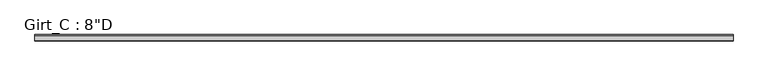
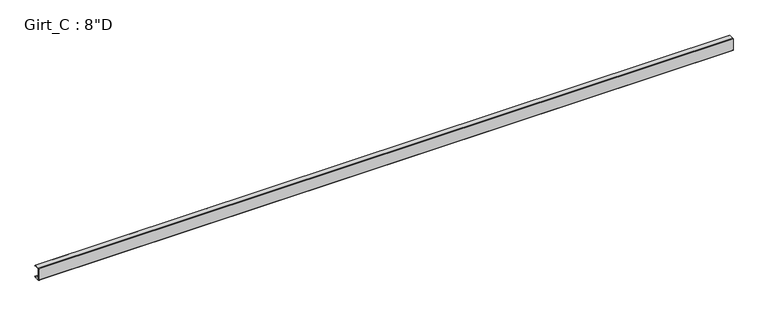
"""IFC4 building model written with IfcOpenShell, lengths in millimetres: beam geometry."""

from ifc_helpers import new_model, si_unit, point, frame, frame_2d, origin, place, context, project, spatial, polyline, circle_curve, trimmed, segment, composite_curve, outline, extrude, source, transform, mapped, element, save


def beam_5935eb23(model_context):
    return source(origin(), model_context, "Body", "SweptSolid", [
        extrude(outline(composite_curve([segment(polyline([(87.5109375, 101.6), (99.7560415, 87.0068534), (97.6278742, 85.221109), (86.2154765, 98.821875), (3.3005807, 98.821875)]), True, "CONTINUOUS"), segment(trimmed(circle_curve(frame_2d((3.3741066, 96.8381931)), 1.9850441), [point((3.3005807, 98.821875))], [point((1.3890625, 96.8381931))], True, "CARTESIAN"), True, "CONTINUOUS"), segment(polyline([(1.3890625, 96.8381931), (1.3890625, -96.8389339)]), True, "CONTINUOUS"), segment(trimmed(circle_curve(frame_2d((3.3748024, -96.8389339)), 1.9857399), [point((1.3890625, -96.8389339))], [point((3.2694106, -98.821875))], True, "CARTESIAN"), True, "CONTINUOUS"), segment(polyline([(3.2694106, -98.821875), (86.2154765, -98.821875), (97.6510975, -85.1934327), (99.7792647, -86.979177), (87.5109375, -101.6), (3.3734375, -101.6)]), True, "CONTINUOUS"), segment(trimmed(circle_curve(frame_2d((3.3734375, -96.8375)), 4.7625), [point((3.3734375, -101.6))], [point((-1.3890625, -96.8375))], False, "CARTESIAN"), True, "CONTINUOUS"), segment(polyline([(-1.3890625, -96.8375), (-1.3890625, 96.8375)]), True, "CONTINUOUS"), segment(trimmed(circle_curve(frame_2d((3.3734375, 96.8375)), 4.7625), [point((-1.3890625, 96.8375))], [point((3.3734375, 101.6))], False, "CARTESIAN"), True, "CONTINUOUS"), segment(polyline([(3.3734375, 101.6), (87.5109375, 101.6)]), True, "CONTINUOUS")], self_intersect=False)), frame((-5621.3960997, 0.0, 0.0), z_axis=(1.0, 0.0, 0.0), x_axis=(0.0, 1.0, 0.0)), (0.0, 0.0, 1.0), 11076.8984495),
    ])


if __name__ == "__main__":
    model = new_model("IFC4")
    model_context = context("Model", 3, world=origin())
    ifc_project = project(units=[si_unit("LENGTHUNIT", "METRE", prefix="MILLI")], contexts=[model_context])
    site = spatial("IfcSite", under=ifc_project)
    building = spatial("IfcBuilding", under=site)
    placement = place(None, origin())
    beam_shape = beam_5935eb23(model_context)
    element("IfcBeam", 1, ObjectType="Girt_C : 8\"D", at=placement, inside=building, context=model_context, shape_type="MappedRepresentation", body=[
        mapped(beam_shape, transform((0.0, 0.0, 0.0), x_axis=(1.0, 0.0, 0.0), y_axis=(0.0, 1.0, 0.0), z_axis=(0.0, 0.0, 1.0))),
    ])
    save(model, "model.ifc")

# Revit data of these elements
# Type "Girt_C : 8\"D"
#   half leg = 0' - 1 3/4"
#   Web_Thickness = 0' - 0 7/64"
#   Length [instance default] = 10' - 0"
#   Leg_1 = 0' - 3 1/2"
#   Height = 0' - 8"
#   Structural Material [instance default] = none
# Element 1 (IfcBeam, "Girt_C : 8\"D")
#   Structural Material = CEE' SECTION (8.0x3.5C - SEE STRUCT. DWGS)
#   Materials on its faces: "CEE' SECTION (8.0x3.5C - SEE STRUCT. DWGS)"
# Materials
#   "CEE' SECTION (8.0x3.5C - SEE STRUCT. DWGS)": class "Metal", colour RGB 137 146 153, transparency 0, Description = "Steel, mill finish", Cost = 0
